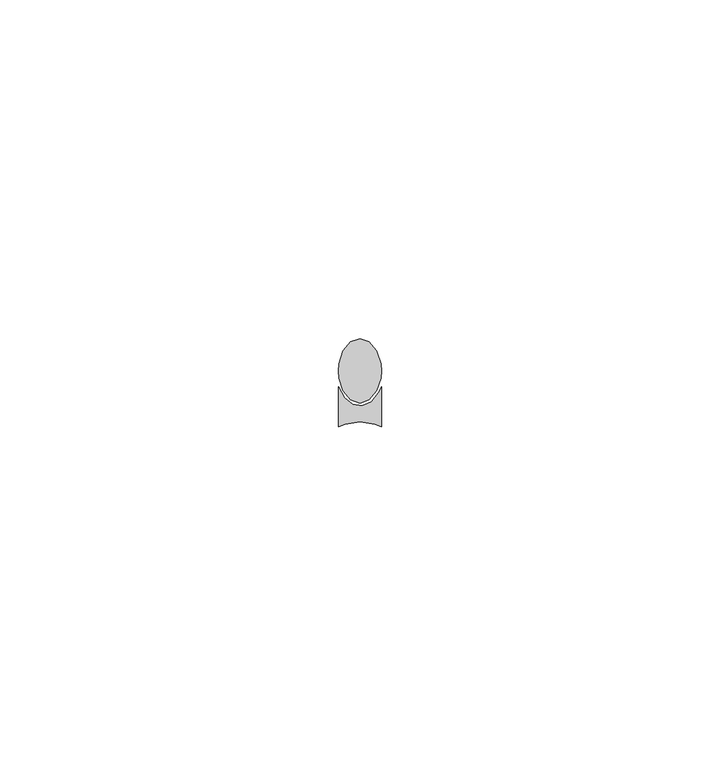
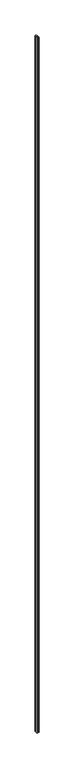
"""IFC4 building model written with IfcOpenShell, lengths in millimetres: proxy geometry, Generic Models 11:Generic Models 1:306267:Generic Models 1:306267 : Generic Models 11:Generic Models 1:306267:300405:Generic Models 1:306267:Generic Models 1:306267 : Generic Models 11:Generic Models 1:306267:300405 : Generic Models 11:Generic Models 1:306267:Generic Models 1:306267 : Generic Models 11:Generic Models 1:306267:300405:33 : Generic Models 11:Generic Models 1:306267:Generic Models 1:306267 : Generic Models 11:Generic Models 1:306267:300405:Generic Models 1:306267:Generic Models 1:306267 : Generic Models 11:Generic Models 1:306267:300405 : Generic Models 11:Generic Models 1:306267:Generic Models 1:306267 : Generic Models 11:Generic Models 1:306267:300405:300182."""

from ifc_helpers import new_model, si_unit, frame, origin, place, context, project, spatial, polyline, outline, extrude, source, transform, mapped, element, save


def generic_models_11c5bab9(model_context):
    return source(origin(), model_context, "Body", "SweptSolid", [
        extrude(outline(polyline([(667547.8021471, -568226.1555576), (667546.4245663, -568226.6271934), (667545.0469854, -568226.1555576), (667543.9422513, -568224.8340636), (667543.3291701, -568222.9244494), (667543.2495663, -568221.8646934), (667543.3291701, -568220.8049375), (667543.9422513, -568218.8953232), (667545.0469854, -568217.5738292), (667546.4245663, -568217.1021934), (667547.8021471, -568217.5738292), (667548.9068812, -568218.8953232), (667549.5199624, -568220.8049375), (667549.5995663, -568221.8646934), (667549.5199624, -568222.9244494), (667548.9068812, -568224.8340636), (667547.8021471, -568226.1555576)])), frame((0.0, 0.0, 6165.85), z_axis=(0.0, 0.0, 1.0), x_axis=(1.0, 0.0, 0.0)), (0.0, 0.0, 1.0), 2412.8015625),
        extrude(outline(polyline([(667544.2153295, -568229.7190045), (667543.2495663, -568230.0964131), (667543.2495663, -568224.228321), (667544.1323551, -568225.8215377), (667545.3737392, -568226.7957427), (667546.7795155, -568226.9985306), (667548.1297632, -568226.3981771), (667549.2132487, -568225.088602), (667549.5995663, -568224.228321), (667549.5995663, -568230.0964131), (667548.633803, -568229.7190045), (667546.4245663, -568229.4053184), (667544.2153295, -568229.7190045)])), frame((0.0, 0.0, 6165.85), z_axis=(0.0, 0.0, 1.0), x_axis=(1.0, 0.0, 0.0)), (0.0, 0.0, 1.0), 2412.8015625),
    ])


if __name__ == "__main__":
    model = new_model("IFC4")
    model_context = context("Model", 3, world=origin())
    ifc_project = project(units=[si_unit("LENGTHUNIT", "METRE", prefix="MILLI")], contexts=[model_context])
    site = spatial("IfcSite", under=ifc_project)
    building = spatial("IfcBuilding", under=site)
    placement = place(None, origin())
    generic_models_shape = generic_models_11c5bab9(model_context)
    element("IfcBuildingElementProxy", 1, Name="Generic Models 11:Generic Models 1:306267:Generic Models 1:306267 : Generic Models 11:Generic Models 1:306267:300405:Generic Models 1:306267:Generic Models 1:306267 : Generic Models 11:Generic Models 1:306267:300405 : Generic Models 11:Generic Models 1:306267:Generic Models 1:306267 : Generic Models 11:Generic Models 1:306267:300405:33 : Generic Models 11:Generic Models 1:306267:Generic Models 1:306267 : Generic Models 11:Generic Models 1:306267:300405:Generic Models 1:306267:Generic Models 1:306267 : Generic Models 11:Generic Models 1:306267:300405 : Generic Models 11:Generic Models 1:306267:Generic Models 1:306267 : Generic Models 11:Generic Models 1:306267:300405:300182", ObjectType="Generic Models 11:Generic Models 1:306267:Generic Models 1:306267 : Generic Models 11:Generic Models 1:306267:300405:Generic Models 1:306267:Generic Models 1:306267 : Generic Models 11:Generic Models 1:306267:300405 : Generic Models 11:Generic Models 1:306267:Generic Models 1:306267 : Generic Models 11:Generic Models 1:306267:300405:33 : Generic Models 11:Generic Models 1:306267:Generic Models 1:306267 : Generic Models 11:Generic Models 1:306267:300405:Generic Models 1:306267:Generic Models 1:306267 : Generic Models 11:Generic Models 1:306267:300405 : Generic Models 11:Generic Models 1:306267:Generic Models 1:306267 : Generic Models 11:Generic Models 1:306267:300405:300182", at=placement, inside=building, context=model_context, shape_type="MappedRepresentation", body=[
        mapped(generic_models_shape, transform((0.0, 0.0, 0.0), x_axis=(1.0, 0.0, 0.0), y_axis=(0.0, 1.0, 0.0), z_axis=(0.0, 0.0, 1.0))),
    ])
    save(model, "model.ifc")

# Revit data of these elements
# Type "Generic Models 11:Generic Models 1:306267:Generic Models 1:306267 : Generic Models 11:Generic Models 1:306267:300405:Generic Models 1:306267:Generic Models 1:306267 : Generic Models 11:Generic Models 1:306267:300405 : Generic Models 11:Generic Models 1:306267:Generic Models 1:306267 : Generic Models 11:Generic Models 1:306267:300405:33 : Generic Models 11:Generic Models 1:306267:Generic Models 1:306267 : Generic Models 11:Generic Models 1:306267:300405:Generic Models 1:306267:Generic Models 1:306267 : Generic Models 11:Generic Models 1:306267:300405 : Generic Models 11:Generic Models 1:306267:Generic Models 1:306267 : Generic Models 11:Generic Models 1:306267:300405:300182"
#   NameOverride = "Generic Models 11:Generic Models 1:306267:Generic Models 1:306267 : Generic Models 11:Generic Models 1:306267:300405:Generic Models 1:306267:Generic Models 1:306267 : Generic Models 11:Generic Models 1:306267:300405 : Generic Models 11:Generic Models 1:306267:Generic Models 1:306267 : Generic Models 11:Generic Models 1:306267:300405:300182"
#   ObjectTypeOverride = "Generic Models 1:306267:Generic Models 1:306267 : Generic Models 11:Generic Models 1:306267:300405 : Generic Models 11:Generic Models 1:306267:Generic Models 1:306267 : Generic Models 11:Generic Models 1:306267:300405"
#   Reference = "Generic Models 1"
#   Tag = "300182"
# Element 1 (IfcBuildingElementProxy, "Generic Models 11:Generic Models 1:306267:Generic Models 1:306267 : Generic Models 11:Generic Models 1:306267:300405:Generic Models 1:306267:Generic Models 1:306267 : Generic Models 11:Generic Models 1:306267:300405 : Generic Models 11:Generic Models 1:306267:Generic Models 1:306267 : Generic Models 11:Generic Models 1:306267:300405:33 : Generic Models 11:Generic Models 1:306267:Generic Models 1:306267 : Generic Models 11:Generic Models 1:306267:300405:Generic Models 1:306267:Generic Models 1:306267 : Generic Models 11:Generic Models 1:306267:300405 : Generic Models 11:Generic Models 1:306267:Generic Models 1:306267 : Generic Models 11:Generic Models 1:306267:300405:300182")
#   Materials on its faces: "SEALANT & BACKER ROD, IF NECESSARY"
# Materials
#   "SEALANT & BACKER ROD, IF NECESSARY": class "Unassigned", colour RGB 120 120 120, transparency 0, Cost = 0
